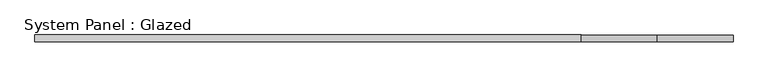
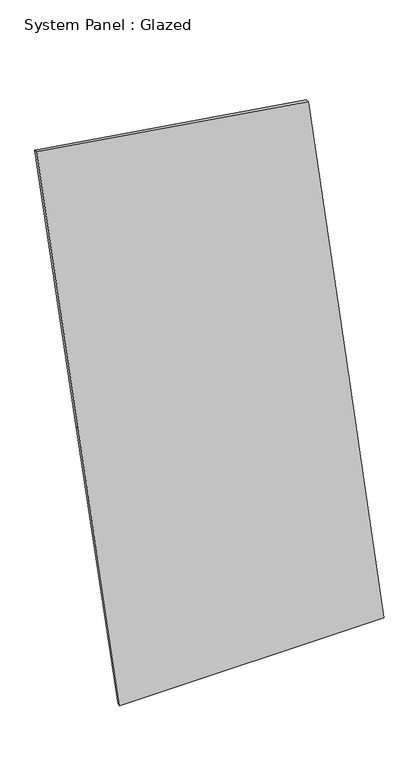
"""IFC4 building model written with IfcOpenShell, lengths in millimetres: plate geometry, System Panel : Glazed."""

from ifc_helpers import new_model, si_unit, frame, origin, place, context, project, spatial, polyline, outline, extrude, source, transform, mapped, element, save


def system_panel_glazed_390c8bc3(model_context):
    return source(origin(), model_context, "Body", "SweptSolid", [
        extrude(outline(polyline([(0.0, -676.1808243), (0.0, 1295.9782327), (2133.6107436, 1014.2371222), (4267.2214872, 732.4960117), (4581.0192528, -1295.9782327), (2290.5096264, -986.0795285), (0.0, -676.1808243)])), frame((0.0, -49.5, 0.0), z_axis=(0.0, 1.0, 0.0), x_axis=(0.0, 0.0, 1.0)), (0.0, 0.0, 1.0), 25.0),
    ])


if __name__ == "__main__":
    model = new_model("IFC4")
    model_context = context("Model", 3, world=origin())
    ifc_project = project(units=[si_unit("LENGTHUNIT", "METRE", prefix="MILLI")], contexts=[model_context])
    site = spatial("IfcSite", under=ifc_project)
    building = spatial("IfcBuilding", under=site)
    placement = place(None, origin())
    system_panel_glazed_shape = system_panel_glazed_390c8bc3(model_context)
    element("IfcPlate", 1, ObjectType="System Panel : Glazed", at=placement, inside=building, context=model_context, shape_type="MappedRepresentation", body=[
        mapped(system_panel_glazed_shape, transform((0.0, 0.0, 0.0), x_axis=(1.0, 0.0, 0.0), y_axis=(0.0, 1.0, 0.0), z_axis=(0.0, 0.0, 1.0))),
    ])
    save(model, "model.ifc")

# Revit data of these elements
# Element 1 (IfcPlate, "System Panel : Glazed")
#   Materials on its faces: "Glass, Clear Glazing"
# Materials
#   "Glass, Clear Glazing": class "Glass", colour RGB 247 249 248, transparency 0.85, Description = "Clear glazing", Cost = 0
